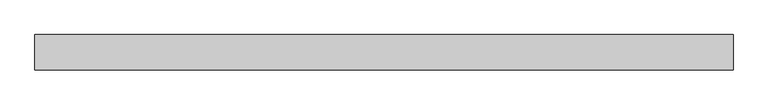
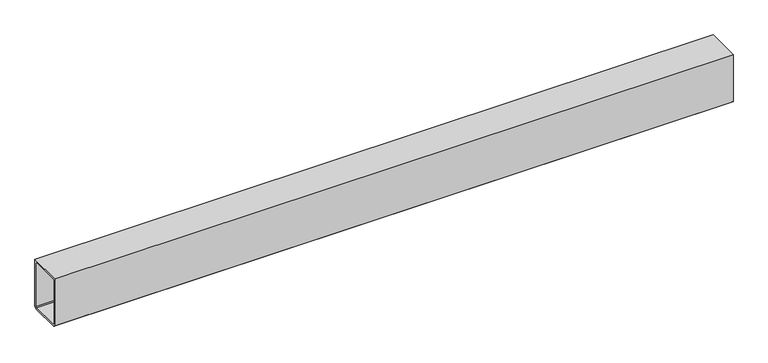
"""IFC4 building model written with IfcOpenShell, lengths in millimetres: proxy geometry, Door frame2:Door frame020:291292 : Door frame2:Door frame020:291292."""

from ifc_helpers import new_model, si_unit, frame, origin, place, context, project, spatial, polyline, outline, extrude, source, transform, mapped, element, save


def generic_models_e8bdbd52(model_context):
    return source(origin(), model_context, "Body", "SweptSolid", [
        extrude(outline(polyline([(9922.714244, 37706.046), (9922.714244, 37852.096), (10024.314244, 37852.096), (10024.314244, 37706.046), (10017.964244, 37699.696), (9929.064244, 37699.696), (9922.714244, 37706.046)]), holes=[polyline([(10015.3339879, 37706.046), (10017.964244, 37708.6762561), (10017.964244, 37843.1157439), (10015.3339879, 37845.746), (9931.6945001, 37845.746), (9929.064244, 37843.1157439), (9929.064244, 37708.6762561), (9931.6945001, 37706.046), (10015.3339879, 37706.046)])]), frame((-4455.0628198, 0.0, 0.0), z_axis=(1.0, 0.0, 0.0), x_axis=(0.0, 1.0, 0.0)), (0.0, 0.0, 1.0), 1999.85),
    ])


if __name__ == "__main__":
    model = new_model("IFC4")
    model_context = context("Model", 3, world=origin())
    ifc_project = project(units=[si_unit("LENGTHUNIT", "METRE", prefix="MILLI")], contexts=[model_context])
    site = spatial("IfcSite", under=ifc_project)
    building = spatial("IfcBuilding", under=site)
    placement = place(None, origin())
    generic_models_shape = generic_models_e8bdbd52(model_context)
    element("IfcBuildingElementProxy", 1, Name="Door frame2:Door frame020:291292 : Door frame2:Door frame020:291292", ObjectType="Door frame2:Door frame020:291292 : Door frame2:Door frame020:291292", at=placement, inside=building, context=model_context, shape_type="MappedRepresentation", body=[
        mapped(generic_models_shape, transform((0.0, 0.0, 0.0), x_axis=(1.0, 0.0, 0.0), y_axis=(0.0, 1.0, 0.0), z_axis=(0.0, 0.0, 1.0))),
    ])
    save(model, "model.ifc")

# Revit data of these elements
# Type "Door frame2:Door frame020:291292 : Door frame2:Door frame020:291292"
#   NameOverride = "Door frame2:Door frame020:291292"
#   ObjectTypeOverride = "Door frame2:Door frame020"
#   Reference = "Door frame020"
#   Category = "Generic Models"
#   Tag = "291292"
# Element 1 (IfcBuildingElementProxy, "Door frame2:Door frame020:291292 : Door frame2:Door frame020:291292")
#   Materials on its faces: "TUBE STEEL PROFILE - METALIZED, PRIMED & PAINTED (COLOR PER ARCHITECT)"
# Materials
#   "TUBE STEEL PROFILE - METALIZED, PRIMED & PAINTED (COLOR PER ARCHITECT)": class "Unassigned", colour RGB 128 128 128, transparency 0
